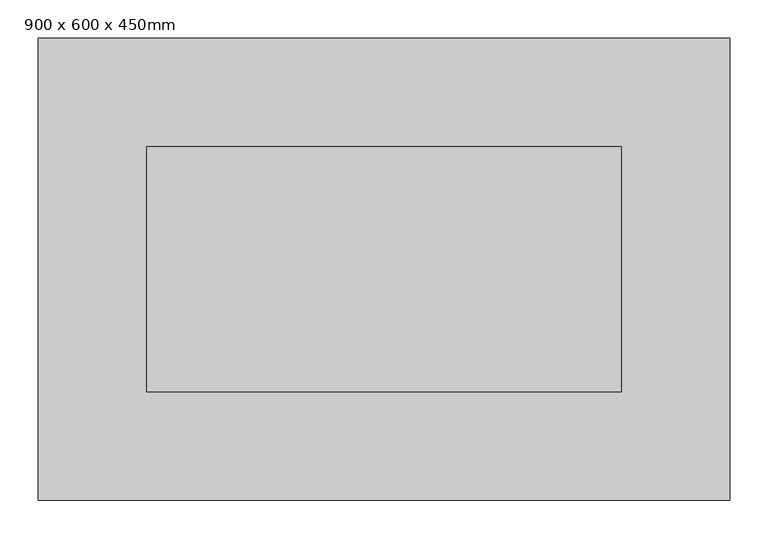
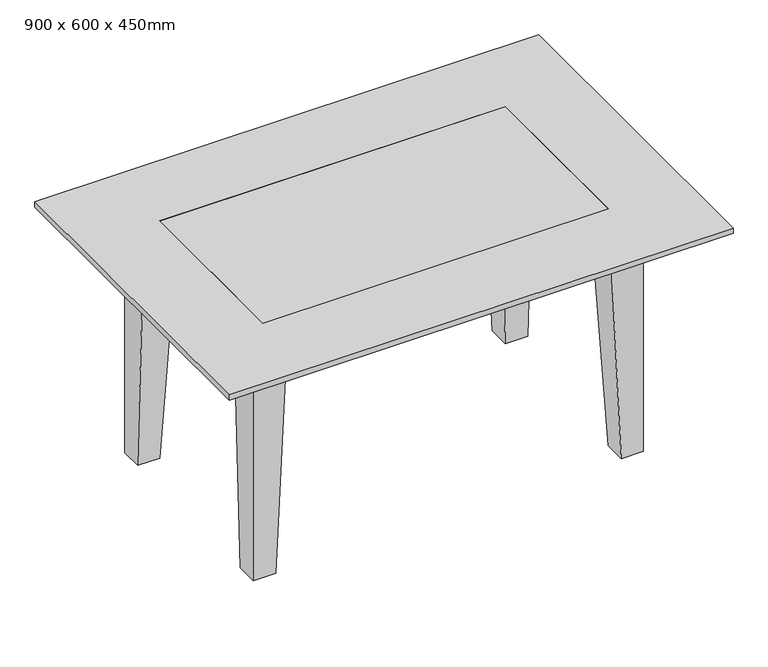
"""IFC4 building model written with IfcOpenShell, lengths in millimetres: furniture geometry, リビングテーブル : 900 x 600 x 450mm."""

import ifcopenshell
import ifcopenshell.guid

model = None  # the IFC model being written
_history = None  # IfcOwnerHistory: only IFC2X3 demands one
_inside = {}  # id of a spatial element -> (the spatial element, [elements in it])
_under = {}  # id of a project, library or spatial element -> (it, [spatial elements below it])
_declared = {}  # id of a project -> (the project, [libraries it declares])
_typed = {}  # id of a type object -> (the type object, [elements of that type])
_made_of = {}  # id of a material, layer set ... -> (it, [elements and type objects made of it])


def new_model(schema):
    """Start an empty IFC model of exactly this schema.

    Asked for "IFC4X3", IfcOpenShell would pick the latest addendum, in which some entities
    have other attributes; the version numbers below select the first issue.
    IFC2X3 requires an IfcOwnerHistory on every rooted entity: one is made here for all.
    """
    global model, _history
    if schema == "IFC4X3":
        model = ifcopenshell.file(schema_version=(4, 3, 0, 0))
    else:
        model = ifcopenshell.file(schema=schema)
    _inside.clear()
    _under.clear()
    _declared.clear()
    _typed.clear()
    _made_of.clear()
    _history = None
    if model.schema == "IFC2X3":
        org = make("IfcOrganization", Name="unknown")
        user = make(
            "IfcPersonAndOrganization",
            ThePerson=make("IfcPerson", FamilyName="unknown"),
            TheOrganization=org,
        )
        app = make(
            "IfcApplication",
            ApplicationDeveloper=org,
            Version="unknown",
            ApplicationFullName="unknown",
            ApplicationIdentifier="unknown",
        )
        _history = make(
            "IfcOwnerHistory",
            OwningUser=user,
            OwningApplication=app,
            ChangeAction="ADDED",
            CreationDate=0,
        )
    return model


def make(cls, **values):
    """One entity of the class cls with the attributes given. An attribute that is None is left unset."""
    return model.create_entity(
        cls, **{name: value for name, value in values.items() if value is not None}
    )


def rooted(cls, **values):
    """An entity with a GlobalId (a new one), such as an element, a storey or a relation."""
    return make(cls, GlobalId=ifcopenshell.guid.new(), OwnerHistory=_history, **values)


def si_unit(unit_type, name, prefix=None):
    """IfcSIUnit, for example si_unit("LENGTHUNIT", "METRE", prefix="MILLI")."""
    return make("IfcSIUnit", UnitType=unit_type, Prefix=prefix, Name=name)


def assignment(units):
    """IfcUnitAssignment: the units of a project."""
    return None if units is None else make("IfcUnitAssignment", Units=units)


def point(xyz):
    """IfcCartesianPoint."""
    return None if xyz is None else make("IfcCartesianPoint", Coordinates=xyz)


def direction(xyz):
    """IfcDirection."""
    return None if xyz is None else make("IfcDirection", DirectionRatios=xyz)


def frame(location, z_axis=None, x_axis=None):
    """IfcAxis2Placement3D, a coordinate frame: its origin and axes. An axis left out is left unset."""
    return make(
        "IfcAxis2Placement3D",
        Location=point(location),
        Axis=direction(z_axis),
        RefDirection=direction(x_axis),
    )


def origin():
    """The frame at (0, 0, 0) with its axes left unset."""
    return frame((0.0, 0.0, 0.0))


def place(relative_to, where):
    """IfcLocalPlacement: puts the frame where relative to a parent placement (None: the world)."""
    return make(
        "IfcLocalPlacement", PlacementRelTo=relative_to, RelativePlacement=where
    )


def context(
    kind, dimensions, precision=None, world=None, true_north=None, identifier=None
):
    """IfcGeometricRepresentationContext, for example the 3D "Model" context."""
    return make(
        "IfcGeometricRepresentationContext",
        ContextIdentifier=identifier,
        ContextType=kind,
        CoordinateSpaceDimension=dimensions,
        Precision=precision,
        WorldCoordinateSystem=world,
        TrueNorth=true_north,
    )


def project(units=None, contexts=None):
    """IfcProject with its units and contexts."""
    return rooted(
        "IfcProject",
        Name="project",
        RepresentationContexts=contexts,
        UnitsInContext=assignment(units),
    )


def spatial(cls, under=None, at=None, **own):
    """A site, building, storey or space (cls), placed at a placement, below another one or the project."""
    s = rooted(cls, ObjectPlacement=at, **own)
    if under is not None:
        _under.setdefault(under.id(), (under, []))[1].append(s)
    return s


def polyline(points):
    """IfcPolyline through the points."""
    return make("IfcPolyline", Points=[point(p) for p in points])


def outline(outer, holes=None, kind="AREA"):
    """IfcArbitraryClosedProfileDef: a profile drawn as a closed curve; with holes, ...WithVoids."""
    if holes is None:
        return make("IfcArbitraryClosedProfileDef", ProfileType=kind, OuterCurve=outer)
    return make(
        "IfcArbitraryProfileDefWithVoids",
        ProfileType=kind,
        OuterCurve=outer,
        InnerCurves=holes,
    )


def extrude(swept, where, along, depth):
    """IfcExtrudedAreaSolid: the profile swept, set in the frame where, extruded along a direction by depth."""
    return make(
        "IfcExtrudedAreaSolid",
        SweptArea=swept,
        Position=where,
        ExtrudedDirection=direction(along),
        Depth=depth,
    )


def faces_of(points, faces, orient=None, outer=None):
    """IfcFace entities. A face is a list of loops; a loop is a list of indices into points, from 0.

    orient and outer hold one flag for each loop. By default every Orientation is true, the
    first loop of a face is its IfcFaceOuterBound and the others are IfcFaceBound.
    """
    made = []
    for i, loops in enumerate(faces):
        bounds = []
        for j, loop in enumerate(loops):
            is_outer = j == 0 if outer is None else outer[i][j]
            bounds.append(
                make(
                    "IfcFaceOuterBound" if is_outer else "IfcFaceBound",
                    Bound=make("IfcPolyLoop", Polygon=[points[k] for k in loop]),
                    Orientation=True if orient is None else orient[i][j],
                )
            )
        made.append(make("IfcFace", Bounds=bounds))
    return made


def faceted_brep(points, faces, orient=None, outer=None, voids=None):
    """IfcFacetedBrep: a solid bounded by flat faces; with voids (closed shells), ...WithVoids."""
    shared = [point(p) for p in points]
    hull = make("IfcClosedShell", CfsFaces=faces_of(shared, faces, orient, outer))
    if voids is None:
        return make("IfcFacetedBrep", Outer=hull)
    return make(
        "IfcFacetedBrepWithVoids",
        Outer=hull,
        Voids=[
            make(cls, CfsFaces=faces_of(shared, fs, o, b)) for cls, fs, o, b in voids
        ],
    )


def shape(context_of_items, identifier, shape_type, items):
    """IfcShapeRepresentation: the items that make up one representation, for example the "Body"."""
    return make(
        "IfcShapeRepresentation",
        ContextOfItems=context_of_items,
        RepresentationIdentifier=identifier,
        RepresentationType=shape_type,
        Items=items,
    )


def source(mapping_origin, context_of_items, identifier, shape_type, items):
    """IfcRepresentationMap: a shape defined once, which mapped items show again and again."""
    return make(
        "IfcRepresentationMap",
        MappingOrigin=mapping_origin,
        MappedRepresentation=shape(context_of_items, identifier, shape_type, items),
    )


def transform(
    local_origin,
    x_axis=None,
    y_axis=None,
    z_axis=None,
    scale=None,
    scale2=None,
    scale3=None,
    uniform=True,
):
    """IfcCartesianTransformationOperator3D, or its non-uniform kind. x_axis, y_axis, z_axis: its Axis1, 2, 3."""
    if uniform:
        return make(
            "IfcCartesianTransformationOperator3D",
            Axis1=direction(x_axis),
            Axis2=direction(y_axis),
            LocalOrigin=point(local_origin),
            Scale=scale,
            Axis3=direction(z_axis),
        )
    return make(
        "IfcCartesianTransformationOperator3DnonUniform",
        Axis1=direction(x_axis),
        Axis2=direction(y_axis),
        LocalOrigin=point(local_origin),
        Scale=scale,
        Axis3=direction(z_axis),
        Scale2=scale2,
        Scale3=scale3,
    )


def mapped(mapping_source, mapping_target):
    """IfcMappedItem: shows the shape of a source again, moved by a transform."""
    return make(
        "IfcMappedItem", MappingSource=mapping_source, MappingTarget=mapping_target
    )


def made_of(thing, what):
    """Note that an element or type object is made of a material, layer set ...; save() writes the relation."""
    if what is not None:
        _made_of.setdefault(what.id(), (what, []))[1].append(thing)
    return thing


def element(
    cls,
    number,
    at=None,
    inside=None,
    cuts=None,
    type_object=None,
    material=None,
    context=None,
    identifier="Body",
    shape_type=None,
    held_by="IfcProductDefinitionShape",
    body=None,
    shapes=None,
    **own,
):
    """One element of the class cls, such as IfcWall. Its Tag is "e" and its number.

    at: its placement. inside: the storey or other place that contains it. cuts: it is an
    opening in that element (IfcRelVoidsElement). A single representation is given by context,
    identifier, shape_type and body (its items); several are given by shapes. held_by: the class
    of the entity that holds the representations. save() writes the other relations.
    """
    e = rooted(cls, Tag="e%d" % number, ObjectPlacement=at, **own)
    if body is not None:
        shapes = [shape(context, identifier, shape_type, body)]
    if shapes is not None:
        e.Representation = make(held_by, Representations=shapes)
    if inside is not None:
        _inside.setdefault(inside.id(), (inside, []))[1].append(e)
    if cuts is not None:
        rooted(
            "IfcRelVoidsElement", RelatingBuildingElement=cuts, RelatedOpeningElement=e
        )
    if type_object is not None:
        _typed.setdefault(type_object.id(), (type_object, []))[1].append(e)
    return made_of(e, material)


def aggregate(whole, parts):
    """IfcRelAggregates: a whole, such as a stair, and the parts it consists of."""
    return rooted("IfcRelAggregates", RelatingObject=whole, RelatedObjects=parts)


def save(model, path):
    """Write the relations noted so far, then the file.

    IfcRelAggregates (storeys below a building ...), IfcRelContainedInSpatialStructure (elements
    in a storey), IfcRelDefinesByType, IfcRelAssociatesMaterial and IfcRelDeclares: one each for
    every whole, place, type object, material and project.
    """
    for whole, parts in _under.values():
        aggregate(whole, parts)
    for where, things in _inside.values():
        rooted(
            "IfcRelContainedInSpatialStructure",
            RelatedElements=things,
            RelatingStructure=where,
        )
    for kind, things in _typed.values():
        rooted("IfcRelDefinesByType", RelatedObjects=things, RelatingType=kind)
    for what, things in _made_of.values():
        rooted("IfcRelAssociatesMaterial", RelatedObjects=things, RelatingMaterial=what)
    for by, libraries in _declared.values():
        rooted("IfcRelDeclares", RelatingContext=by, RelatedDefinitions=libraries)
    model.write(path)


def furniture_900_x_600_x_450mm_e2215332(model_context):
    return source(origin(), model_context, "Body", "SolidModel", [
        extrude(outline(polyline([(330.0, 180.0), (330.0, -180.0), (-330.0, -180.0), (-330.0, 180.0), (330.0, 180.0)]), holes=[polyline([(290.0, 140.0), (-290.0, 140.0), (-290.0, -140.0), (290.0, -140.0), (290.0, 140.0)])]), frame((0.0, 0.0, 360.0), z_axis=(0.0, 0.0, 1.0), x_axis=(1.0, 0.0, 0.0)), (0.0, 0.0, 1.0), 60.0),
        faceted_brep([(452.0830728, 302.0830728, 440.0), (452.0830728, 302.0830728, 450.0), (452.0830728, -302.0830728, 450.0), (452.0830728, -302.0830728, 440.0), (350.0, 200.0, 420.0), (350.0, -200.0, 420.0), (310.0, 160.0, 450.0), (310.0, 160.0, 420.0), (310.0, -160.0, 420.0), (310.0, -160.0, 450.0), (-452.0830728, -302.0830728, 450.0), (-452.0830728, -302.0830728, 440.0), (-350.0, -200.0, 420.0), (-310.0, -160.0, 420.0), (-310.0, -160.0, 450.0), (-452.0830728, 302.0830728, 450.0), (-452.0830728, 302.0830728, 440.0), (-350.0, 200.0, 420.0), (-310.0, 160.0, 420.0), (-310.0, 160.0, 450.0)], [[[0, 1, 2, 3]], [[4, 0, 3, 5]], [[6, 7, 8, 9]], [[3, 2, 10, 11]], [[5, 3, 11, 12]], [[9, 8, 13, 14]], [[11, 10, 15, 16]], [[12, 11, 16, 17]], [[14, 13, 18, 19]], [[16, 15, 1, 0]], [[17, 16, 0, 4]], [[5, 12, 17, 4], [7, 18, 13, 8]], [[19, 18, 7, 6]], [[1, 15, 10, 2], [9, 14, 19, 6]]]),
        extrude(outline(polyline([(310.0, 160.0), (310.0, -160.0), (-310.0, -160.0), (-310.0, 160.0), (310.0, 160.0)])), frame((0.0, 0.0, 420.0), z_axis=(0.0, 0.0, 1.0), x_axis=(1.0, 0.0, 0.0)), (0.0, 0.0, 1.0), 30.0),
        faceted_brep([(-290.0, -200.0, 420.0), (-290.0, -139.9690818, 420.0), (-350.0, -139.9690818, 420.0), (-350.0, -200.0, 420.0), (-310.0, -200.0, 0.0), (-350.0, -200.0, 0.0), (-350.0, -160.0, 0.0), (-310.0, -160.0, 0.0)], [[[0, 1, 2, 3]], [[4, 5, 6, 7]], [[1, 0, 4, 7]], [[2, 1, 7, 6]], [[3, 2, 6, 5]], [[0, 3, 5, 4]]]),
        faceted_brep([(-290.0, 200.0, 420.0), (-350.0, 200.0, 420.0), (-350.0, 139.9690818, 420.0), (-290.0, 139.9690818, 420.0), (-310.0, 200.0, 0.0), (-310.0, 160.0, 0.0), (-350.0, 160.0, 0.0), (-350.0, 200.0, 0.0)], [[[0, 1, 2, 3]], [[4, 5, 6, 7]], [[1, 0, 4, 7]], [[2, 1, 7, 6]], [[3, 2, 6, 5]], [[0, 3, 5, 4]]]),
        faceted_brep([(290.0, -200.0, 420.0), (350.0, -200.0, 420.0), (350.0, -139.9690818, 420.0), (290.0, -139.9690818, 420.0), (310.0, -200.0, 0.0), (310.0, -160.0, 0.0), (350.0, -160.0, 0.0), (350.0, -200.0, 0.0)], [[[0, 1, 2, 3]], [[4, 5, 6, 7]], [[1, 0, 4, 7]], [[2, 1, 7, 6]], [[3, 2, 6, 5]], [[0, 3, 5, 4]]]),
        faceted_brep([(290.0, 200.0, 420.0), (290.0, 139.9690818, 420.0), (350.0, 139.9690818, 420.0), (350.0, 200.0, 420.0), (310.0, 200.0, 0.0), (350.0, 200.0, 0.0), (350.0, 160.0, 0.0), (310.0, 160.0, 0.0)], [[[0, 1, 2, 3]], [[4, 5, 6, 7]], [[1, 0, 4, 7]], [[2, 1, 7, 6]], [[3, 2, 6, 5]], [[0, 3, 5, 4]]]),
    ])


if __name__ == "__main__":
    model = new_model("IFC4")
    model_context = context("Model", 3, world=origin())
    ifc_project = project(units=[si_unit("LENGTHUNIT", "METRE", prefix="MILLI")], contexts=[model_context])
    site = spatial("IfcSite", under=ifc_project)
    building = spatial("IfcBuilding", under=site)
    placement = place(None, origin())
    furniture_900_x_600_x_450mm_shape = furniture_900_x_600_x_450mm_e2215332(model_context)
    element("IfcFurniture", 1, ObjectType="リビングテーブル : 900 x 600 x 450mm", at=placement, inside=building, context=model_context, shape_type="MappedRepresentation", body=[
        mapped(furniture_900_x_600_x_450mm_shape, transform((0.0, 0.0, 0.0), x_axis=(1.0, 0.0, 0.0), y_axis=(0.0, 1.0, 0.0), z_axis=(0.0, 0.0, 1.0))),
    ])
    save(model, "model.ifc")

# Revit data of these elements
# Type "リビングテーブル : 900 x 600 x 450mm"
#   Keynote = "12490.HH1"
#   高さ = 450 mm
#   幅 = 900 mm
#   奥行き = 600 mm
#   本体 = 木目 - ナチュラル
#   天板内側 = 木目 - ミディアムブラウン
#   Default Elevation = 0
# Element 1 (IfcFurniture, "リビングテーブル : 900 x 600 x 450mm")
#   Materials on its faces: "木目 - ナチュラル", "木目 - ミディアムブラウン"
# Materials
#   "木目 - ナチュラル": class "木材", colour RGB 204 173 122, transparency 0, Cost = 0
#   "木目 - ミディアムブラウン": class "木材", colour RGB 102 44 16, transparency 0, Cost = 0
